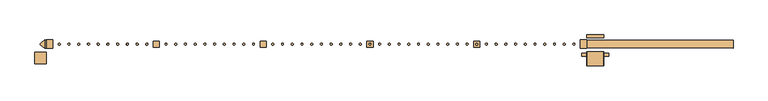
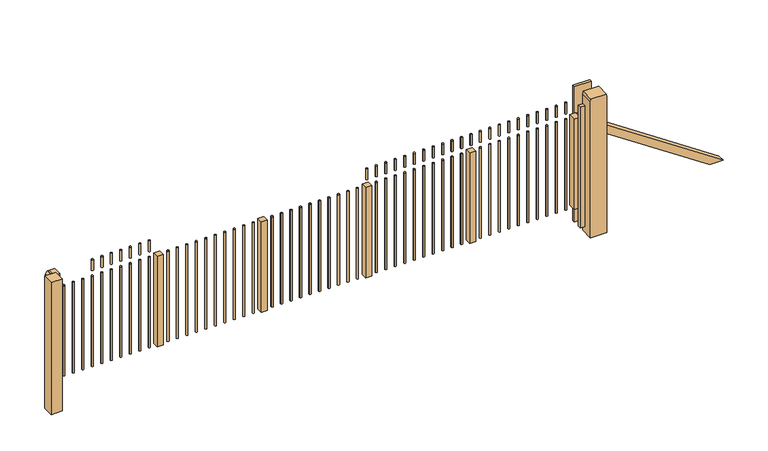
"""IFC4 building model written with IfcOpenShell, lengths in millimetres: door geometry, NLRS_90_DO_UN_schuifpoort met spijlen_gen_rsf : schuifpoort automatisch bxh 7000x1800-NP."""

import ifcopenshell
import ifcopenshell.guid

model = None  # the IFC model being written
_history = None  # IfcOwnerHistory: only IFC2X3 demands one
_inside = {}  # id of a spatial element -> (the spatial element, [elements in it])
_under = {}  # id of a project, library or spatial element -> (it, [spatial elements below it])
_declared = {}  # id of a project -> (the project, [libraries it declares])
_typed = {}  # id of a type object -> (the type object, [elements of that type])
_made_of = {}  # id of a material, layer set ... -> (it, [elements and type objects made of it])


def new_model(schema):
    """Start an empty IFC model of exactly this schema.

    Asked for "IFC4X3", IfcOpenShell would pick the latest addendum, in which some entities
    have other attributes; the version numbers below select the first issue.
    IFC2X3 requires an IfcOwnerHistory on every rooted entity: one is made here for all.
    """
    global model, _history
    if schema == "IFC4X3":
        model = ifcopenshell.file(schema_version=(4, 3, 0, 0))
    else:
        model = ifcopenshell.file(schema=schema)
    _inside.clear()
    _under.clear()
    _declared.clear()
    _typed.clear()
    _made_of.clear()
    _history = None
    if model.schema == "IFC2X3":
        org = make("IfcOrganization", Name="unknown")
        user = make(
            "IfcPersonAndOrganization",
            ThePerson=make("IfcPerson", FamilyName="unknown"),
            TheOrganization=org,
        )
        app = make(
            "IfcApplication",
            ApplicationDeveloper=org,
            Version="unknown",
            ApplicationFullName="unknown",
            ApplicationIdentifier="unknown",
        )
        _history = make(
            "IfcOwnerHistory",
            OwningUser=user,
            OwningApplication=app,
            ChangeAction="ADDED",
            CreationDate=0,
        )
    return model


def make(cls, **values):
    """One entity of the class cls with the attributes given. An attribute that is None is left unset."""
    return model.create_entity(
        cls, **{name: value for name, value in values.items() if value is not None}
    )


def rooted(cls, **values):
    """An entity with a GlobalId (a new one), such as an element, a storey or a relation."""
    return make(cls, GlobalId=ifcopenshell.guid.new(), OwnerHistory=_history, **values)


def si_unit(unit_type, name, prefix=None):
    """IfcSIUnit, for example si_unit("LENGTHUNIT", "METRE", prefix="MILLI")."""
    return make("IfcSIUnit", UnitType=unit_type, Prefix=prefix, Name=name)


def assignment(units):
    """IfcUnitAssignment: the units of a project."""
    return None if units is None else make("IfcUnitAssignment", Units=units)


def point(xyz):
    """IfcCartesianPoint."""
    return None if xyz is None else make("IfcCartesianPoint", Coordinates=xyz)


def direction(xyz):
    """IfcDirection."""
    return None if xyz is None else make("IfcDirection", DirectionRatios=xyz)


def frame(location, z_axis=None, x_axis=None):
    """IfcAxis2Placement3D, a coordinate frame: its origin and axes. An axis left out is left unset."""
    return make(
        "IfcAxis2Placement3D",
        Location=point(location),
        Axis=direction(z_axis),
        RefDirection=direction(x_axis),
    )


def frame_2d(location, x_axis=None):
    """IfcAxis2Placement2D, a coordinate frame in the plane: its origin and x axis."""
    return make(
        "IfcAxis2Placement2D", Location=point(location), RefDirection=direction(x_axis)
    )


def origin():
    """The frame at (0, 0, 0) with its axes left unset."""
    return frame((0.0, 0.0, 0.0))


def place(relative_to, where):
    """IfcLocalPlacement: puts the frame where relative to a parent placement (None: the world)."""
    return make(
        "IfcLocalPlacement", PlacementRelTo=relative_to, RelativePlacement=where
    )


def context(
    kind, dimensions, precision=None, world=None, true_north=None, identifier=None
):
    """IfcGeometricRepresentationContext, for example the 3D "Model" context."""
    return make(
        "IfcGeometricRepresentationContext",
        ContextIdentifier=identifier,
        ContextType=kind,
        CoordinateSpaceDimension=dimensions,
        Precision=precision,
        WorldCoordinateSystem=world,
        TrueNorth=true_north,
    )


def project(units=None, contexts=None):
    """IfcProject with its units and contexts."""
    return rooted(
        "IfcProject",
        Name="project",
        RepresentationContexts=contexts,
        UnitsInContext=assignment(units),
    )


def spatial(cls, under=None, at=None, **own):
    """A site, building, storey or space (cls), placed at a placement, below another one or the project."""
    s = rooted(cls, ObjectPlacement=at, **own)
    if under is not None:
        _under.setdefault(under.id(), (under, []))[1].append(s)
    return s


def polyline(points):
    """IfcPolyline through the points."""
    return make("IfcPolyline", Points=[point(p) for p in points])


def circle_curve(where, radius):
    """IfcCircle in the frame where."""
    return make("IfcCircle", Position=where, Radius=radius)


def trimmed(basis, trim1, trim2, sense, master):
    """IfcTrimmedCurve: the piece of a basis curve between two trims."""
    return make(
        "IfcTrimmedCurve",
        BasisCurve=basis,
        Trim1=trim1,
        Trim2=trim2,
        SenseAgreement=sense,
        MasterRepresentation=master,
    )


def segment(curve, same_sense, transition):
    """IfcCompositeCurveSegment."""
    return make(
        "IfcCompositeCurveSegment",
        Transition=transition,
        SameSense=same_sense,
        ParentCurve=curve,
    )


def composite_curve(segments, self_intersect=None):
    """IfcCompositeCurve: segments joined end to end."""
    return make("IfcCompositeCurve", Segments=segments, SelfIntersect=self_intersect)


def outline(outer, holes=None, kind="AREA"):
    """IfcArbitraryClosedProfileDef: a profile drawn as a closed curve; with holes, ...WithVoids."""
    if holes is None:
        return make("IfcArbitraryClosedProfileDef", ProfileType=kind, OuterCurve=outer)
    return make(
        "IfcArbitraryProfileDefWithVoids",
        ProfileType=kind,
        OuterCurve=outer,
        InnerCurves=holes,
    )


def extrude(swept, where, along, depth):
    """IfcExtrudedAreaSolid: the profile swept, set in the frame where, extruded along a direction by depth."""
    return make(
        "IfcExtrudedAreaSolid",
        SweptArea=swept,
        Position=where,
        ExtrudedDirection=direction(along),
        Depth=depth,
    )


def shape(context_of_items, identifier, shape_type, items):
    """IfcShapeRepresentation: the items that make up one representation, for example the "Body"."""
    return make(
        "IfcShapeRepresentation",
        ContextOfItems=context_of_items,
        RepresentationIdentifier=identifier,
        RepresentationType=shape_type,
        Items=items,
    )


def source(mapping_origin, context_of_items, identifier, shape_type, items):
    """IfcRepresentationMap: a shape defined once, which mapped items show again and again."""
    return make(
        "IfcRepresentationMap",
        MappingOrigin=mapping_origin,
        MappedRepresentation=shape(context_of_items, identifier, shape_type, items),
    )


def transform(
    local_origin,
    x_axis=None,
    y_axis=None,
    z_axis=None,
    scale=None,
    scale2=None,
    scale3=None,
    uniform=True,
):
    """IfcCartesianTransformationOperator3D, or its non-uniform kind. x_axis, y_axis, z_axis: its Axis1, 2, 3."""
    if uniform:
        return make(
            "IfcCartesianTransformationOperator3D",
            Axis1=direction(x_axis),
            Axis2=direction(y_axis),
            LocalOrigin=point(local_origin),
            Scale=scale,
            Axis3=direction(z_axis),
        )
    return make(
        "IfcCartesianTransformationOperator3DnonUniform",
        Axis1=direction(x_axis),
        Axis2=direction(y_axis),
        LocalOrigin=point(local_origin),
        Scale=scale,
        Axis3=direction(z_axis),
        Scale2=scale2,
        Scale3=scale3,
    )


def mapped(mapping_source, mapping_target):
    """IfcMappedItem: shows the shape of a source again, moved by a transform."""
    return make(
        "IfcMappedItem", MappingSource=mapping_source, MappingTarget=mapping_target
    )


def made_of(thing, what):
    """Note that an element or type object is made of a material, layer set ...; save() writes the relation."""
    if what is not None:
        _made_of.setdefault(what.id(), (what, []))[1].append(thing)
    return thing


def element(
    cls,
    number,
    at=None,
    inside=None,
    cuts=None,
    type_object=None,
    material=None,
    context=None,
    identifier="Body",
    shape_type=None,
    held_by="IfcProductDefinitionShape",
    body=None,
    shapes=None,
    **own,
):
    """One element of the class cls, such as IfcWall. Its Tag is "e" and its number.

    at: its placement. inside: the storey or other place that contains it. cuts: it is an
    opening in that element (IfcRelVoidsElement). A single representation is given by context,
    identifier, shape_type and body (its items); several are given by shapes. held_by: the class
    of the entity that holds the representations. save() writes the other relations.
    """
    e = rooted(cls, Tag="e%d" % number, ObjectPlacement=at, **own)
    if body is not None:
        shapes = [shape(context, identifier, shape_type, body)]
    if shapes is not None:
        e.Representation = make(held_by, Representations=shapes)
    if inside is not None:
        _inside.setdefault(inside.id(), (inside, []))[1].append(e)
    if cuts is not None:
        rooted(
            "IfcRelVoidsElement", RelatingBuildingElement=cuts, RelatedOpeningElement=e
        )
    if type_object is not None:
        _typed.setdefault(type_object.id(), (type_object, []))[1].append(e)
    return made_of(e, material)


def aggregate(whole, parts):
    """IfcRelAggregates: a whole, such as a stair, and the parts it consists of."""
    return rooted("IfcRelAggregates", RelatingObject=whole, RelatedObjects=parts)


def save(model, path):
    """Write the relations noted so far, then the file.

    IfcRelAggregates (storeys below a building ...), IfcRelContainedInSpatialStructure (elements
    in a storey), IfcRelDefinesByType, IfcRelAssociatesMaterial and IfcRelDeclares: one each for
    every whole, place, type object, material and project.
    """
    for whole, parts in _under.values():
        aggregate(whole, parts)
    for where, things in _inside.values():
        rooted(
            "IfcRelContainedInSpatialStructure",
            RelatedElements=things,
            RelatingStructure=where,
        )
    for kind, things in _typed.values():
        rooted("IfcRelDefinesByType", RelatedObjects=things, RelatingType=kind)
    for what, things in _made_of.values():
        rooted("IfcRelAssociatesMaterial", RelatedObjects=things, RelatingMaterial=what)
    for by, libraries in _declared.values():
        rooted("IfcRelDeclares", RelatingContext=by, RelatedDefinitions=libraries)
    model.write(path)


def door_c2b4a2f6(model_context):
    return source(origin(), model_context, "Body", "SweptSolid", [
        extrude(outline(composite_curve([segment(trimmed(circle_curve(frame_2d((3299.5, 0.0)), 12.5), [point((3312.0, 0.0))], [point((3287.0, 0.0))], False, "CARTESIAN"), True, "CONTINUOUS"), segment(trimmed(circle_curve(frame_2d((3299.5, 0.0)), 12.5), [point((3287.0, 0.0))], [point((3312.0, 0.0))], False, "CARTESIAN"), True, "CONTINUOUS")], self_intersect=False)), frame((0.0, 0.0, 300.0), z_axis=(0.0, 0.0, 1.0), x_axis=(1.0, 0.0, 0.0)), (0.0, 0.0, 1.0), 1270.0),
        extrude(outline(composite_curve([segment(trimmed(circle_curve(frame_2d((3173.5, 0.0)), 12.5), [point((3186.0, 0.0))], [point((3161.0, 0.0))], False, "CARTESIAN"), True, "CONTINUOUS"), segment(trimmed(circle_curve(frame_2d((3173.5, 0.0)), 12.5), [point((3161.0, 0.0))], [point((3186.0, 0.0))], False, "CARTESIAN"), True, "CONTINUOUS")], self_intersect=False)), frame((0.0, 0.0, 300.0), z_axis=(0.0, 0.0, 1.0), x_axis=(1.0, 0.0, 0.0)), (0.0, 0.0, 1.0), 1270.0),
        extrude(outline(composite_curve([segment(trimmed(circle_curve(frame_2d((3047.5, 0.0)), 12.5), [point((3060.0, 0.0))], [point((3035.0, 0.0))], False, "CARTESIAN"), True, "CONTINUOUS"), segment(trimmed(circle_curve(frame_2d((3047.5, 0.0)), 12.5), [point((3035.0, 0.0))], [point((3060.0, 0.0))], False, "CARTESIAN"), True, "CONTINUOUS")], self_intersect=False)), frame((0.0, 0.0, 300.0), z_axis=(0.0, 0.0, 1.0), x_axis=(1.0, 0.0, 0.0)), (0.0, 0.0, 1.0), 1270.0),
        extrude(outline(composite_curve([segment(trimmed(circle_curve(frame_2d((2921.5, 0.0)), 12.5), [point((2934.0, 0.0))], [point((2909.0, 0.0))], False, "CARTESIAN"), True, "CONTINUOUS"), segment(trimmed(circle_curve(frame_2d((2921.5, 0.0)), 12.5), [point((2909.0, 0.0))], [point((2934.0, 0.0))], False, "CARTESIAN"), True, "CONTINUOUS")], self_intersect=False)), frame((0.0, 0.0, 300.0), z_axis=(0.0, 0.0, 1.0), x_axis=(1.0, 0.0, 0.0)), (0.0, 0.0, 1.0), 1270.0),
        extrude(outline(composite_curve([segment(trimmed(circle_curve(frame_2d((2795.5, 0.0)), 12.5), [point((2808.0, 0.0))], [point((2783.0, 0.0))], False, "CARTESIAN"), True, "CONTINUOUS"), segment(trimmed(circle_curve(frame_2d((2795.5, 0.0)), 12.5), [point((2783.0, 0.0))], [point((2808.0, 0.0))], False, "CARTESIAN"), True, "CONTINUOUS")], self_intersect=False)), frame((0.0, 0.0, 300.0), z_axis=(0.0, 0.0, 1.0), x_axis=(1.0, 0.0, 0.0)), (0.0, 0.0, 1.0), 1270.0),
        extrude(outline(composite_curve([segment(trimmed(circle_curve(frame_2d((2669.5, 0.0)), 12.5), [point((2682.0, 0.0))], [point((2657.0, 0.0))], False, "CARTESIAN"), True, "CONTINUOUS"), segment(trimmed(circle_curve(frame_2d((2669.5, 0.0)), 12.5), [point((2657.0, 0.0))], [point((2682.0, 0.0))], False, "CARTESIAN"), True, "CONTINUOUS")], self_intersect=False)), frame((0.0, 0.0, 300.0), z_axis=(0.0, 0.0, 1.0), x_axis=(1.0, 0.0, 0.0)), (0.0, 0.0, 1.0), 1270.0),
        extrude(outline(composite_curve([segment(trimmed(circle_curve(frame_2d((2543.5, 0.0)), 12.5), [point((2556.0, 0.0))], [point((2531.0, 0.0))], False, "CARTESIAN"), True, "CONTINUOUS"), segment(trimmed(circle_curve(frame_2d((2543.5, 0.0)), 12.5), [point((2531.0, 0.0))], [point((2556.0, 0.0))], False, "CARTESIAN"), True, "CONTINUOUS")], self_intersect=False)), frame((0.0, 0.0, 300.0), z_axis=(0.0, 0.0, 1.0), x_axis=(1.0, 0.0, 0.0)), (0.0, 0.0, 1.0), 1270.0),
        extrude(outline(composite_curve([segment(trimmed(circle_curve(frame_2d((2417.5, 0.0)), 12.5), [point((2430.0, 0.0))], [point((2405.0, 0.0))], False, "CARTESIAN"), True, "CONTINUOUS"), segment(trimmed(circle_curve(frame_2d((2417.5, 0.0)), 12.5), [point((2405.0, 0.0))], [point((2430.0, 0.0))], False, "CARTESIAN"), True, "CONTINUOUS")], self_intersect=False)), frame((0.0, 0.0, 300.0), z_axis=(0.0, 0.0, 1.0), x_axis=(1.0, 0.0, 0.0)), (0.0, 0.0, 1.0), 1270.0),
        extrude(outline(composite_curve([segment(trimmed(circle_curve(frame_2d((2291.5, 0.0)), 12.5), [point((2304.0, 0.0))], [point((2279.0, 0.0))], False, "CARTESIAN"), True, "CONTINUOUS"), segment(trimmed(circle_curve(frame_2d((2291.5, 0.0)), 12.5), [point((2279.0, 0.0))], [point((2304.0, 0.0))], False, "CARTESIAN"), True, "CONTINUOUS")], self_intersect=False)), frame((0.0, 0.0, 300.0), z_axis=(0.0, 0.0, 1.0), x_axis=(1.0, 0.0, 0.0)), (0.0, 0.0, 1.0), 1270.0),
        extrude(outline(composite_curve([segment(trimmed(circle_curve(frame_2d((2165.5, 0.0)), 12.5), [point((2178.0, 0.0))], [point((2153.0, 0.0))], False, "CARTESIAN"), True, "CONTINUOUS"), segment(trimmed(circle_curve(frame_2d((2165.5, 0.0)), 12.5), [point((2153.0, 0.0))], [point((2178.0, 0.0))], False, "CARTESIAN"), True, "CONTINUOUS")], self_intersect=False)), frame((0.0, 0.0, 300.0), z_axis=(0.0, 0.0, 1.0), x_axis=(1.0, 0.0, 0.0)), (0.0, 0.0, 1.0), 1270.0),
        extrude(outline(composite_curve([segment(trimmed(circle_curve(frame_2d((1915.5, 0.0)), 12.5), [point((1928.0, 0.0))], [point((1903.0, 0.0))], False, "CARTESIAN"), True, "CONTINUOUS"), segment(trimmed(circle_curve(frame_2d((1915.5, 0.0)), 12.5), [point((1903.0, 0.0))], [point((1928.0, 0.0))], False, "CARTESIAN"), True, "CONTINUOUS")], self_intersect=False)), frame((0.0, 0.0, 300.0), z_axis=(0.0, 0.0, 1.0), x_axis=(1.0, 0.0, 0.0)), (0.0, 0.0, 1.0), 1270.0),
        extrude(outline(composite_curve([segment(trimmed(circle_curve(frame_2d((1789.5, 0.0)), 12.5), [point((1802.0, 0.0))], [point((1777.0, 0.0))], False, "CARTESIAN"), True, "CONTINUOUS"), segment(trimmed(circle_curve(frame_2d((1789.5, 0.0)), 12.5), [point((1777.0, 0.0))], [point((1802.0, 0.0))], False, "CARTESIAN"), True, "CONTINUOUS")], self_intersect=False)), frame((0.0, 0.0, 300.0), z_axis=(0.0, 0.0, 1.0), x_axis=(1.0, 0.0, 0.0)), (0.0, 0.0, 1.0), 1270.0),
        extrude(outline(composite_curve([segment(trimmed(circle_curve(frame_2d((1663.5, 0.0)), 12.5), [point((1676.0, 0.0))], [point((1651.0, 0.0))], False, "CARTESIAN"), True, "CONTINUOUS"), segment(trimmed(circle_curve(frame_2d((1663.5, 0.0)), 12.5), [point((1651.0, 0.0))], [point((1676.0, 0.0))], False, "CARTESIAN"), True, "CONTINUOUS")], self_intersect=False)), frame((0.0, 0.0, 300.0), z_axis=(0.0, 0.0, 1.0), x_axis=(1.0, 0.0, 0.0)), (0.0, 0.0, 1.0), 1270.0),
        extrude(outline(composite_curve([segment(trimmed(circle_curve(frame_2d((1537.5, 0.0)), 12.5), [point((1550.0, 0.0))], [point((1525.0, 0.0))], False, "CARTESIAN"), True, "CONTINUOUS"), segment(trimmed(circle_curve(frame_2d((1537.5, 0.0)), 12.5), [point((1525.0, 0.0))], [point((1550.0, 0.0))], False, "CARTESIAN"), True, "CONTINUOUS")], self_intersect=False)), frame((0.0, 0.0, 300.0), z_axis=(0.0, 0.0, 1.0), x_axis=(1.0, 0.0, 0.0)), (0.0, 0.0, 1.0), 1270.0),
        extrude(outline(composite_curve([segment(trimmed(circle_curve(frame_2d((1411.5, 0.0)), 12.5), [point((1424.0, 0.0))], [point((1399.0, 0.0))], False, "CARTESIAN"), True, "CONTINUOUS"), segment(trimmed(circle_curve(frame_2d((1411.5, 0.0)), 12.5), [point((1399.0, 0.0))], [point((1424.0, 0.0))], False, "CARTESIAN"), True, "CONTINUOUS")], self_intersect=False)), frame((0.0, 0.0, 300.0), z_axis=(0.0, 0.0, 1.0), x_axis=(1.0, 0.0, 0.0)), (0.0, 0.0, 1.0), 1270.0),
        extrude(outline(composite_curve([segment(trimmed(circle_curve(frame_2d((1285.5, 0.0)), 12.5), [point((1298.0, 0.0))], [point((1273.0, 0.0))], False, "CARTESIAN"), True, "CONTINUOUS"), segment(trimmed(circle_curve(frame_2d((1285.5, 0.0)), 12.5), [point((1273.0, 0.0))], [point((1298.0, 0.0))], False, "CARTESIAN"), True, "CONTINUOUS")], self_intersect=False)), frame((0.0, 0.0, 300.0), z_axis=(0.0, 0.0, 1.0), x_axis=(1.0, 0.0, 0.0)), (0.0, 0.0, 1.0), 1270.0),
        extrude(outline(composite_curve([segment(trimmed(circle_curve(frame_2d((1159.5, 0.0)), 12.5), [point((1172.0, 0.0))], [point((1147.0, 0.0))], False, "CARTESIAN"), True, "CONTINUOUS"), segment(trimmed(circle_curve(frame_2d((1159.5, 0.0)), 12.5), [point((1147.0, 0.0))], [point((1172.0, 0.0))], False, "CARTESIAN"), True, "CONTINUOUS")], self_intersect=False)), frame((0.0, 0.0, 300.0), z_axis=(0.0, 0.0, 1.0), x_axis=(1.0, 0.0, 0.0)), (0.0, 0.0, 1.0), 1270.0),
        extrude(outline(composite_curve([segment(trimmed(circle_curve(frame_2d((1033.5, 0.0)), 12.5), [point((1046.0, 0.0))], [point((1021.0, 0.0))], False, "CARTESIAN"), True, "CONTINUOUS"), segment(trimmed(circle_curve(frame_2d((1033.5, 0.0)), 12.5), [point((1021.0, 0.0))], [point((1046.0, 0.0))], False, "CARTESIAN"), True, "CONTINUOUS")], self_intersect=False)), frame((0.0, 0.0, 300.0), z_axis=(0.0, 0.0, 1.0), x_axis=(1.0, 0.0, 0.0)), (0.0, 0.0, 1.0), 1270.0),
        extrude(outline(composite_curve([segment(trimmed(circle_curve(frame_2d((907.5, 0.0)), 12.5), [point((920.0, 0.0))], [point((895.0, 0.0))], False, "CARTESIAN"), True, "CONTINUOUS"), segment(trimmed(circle_curve(frame_2d((907.5, 0.0)), 12.5), [point((895.0, 0.0))], [point((920.0, 0.0))], False, "CARTESIAN"), True, "CONTINUOUS")], self_intersect=False)), frame((0.0, 0.0, 300.0), z_axis=(0.0, 0.0, 1.0), x_axis=(1.0, 0.0, 0.0)), (0.0, 0.0, 1.0), 1270.0),
        extrude(outline(composite_curve([segment(trimmed(circle_curve(frame_2d((781.5, 0.0)), 12.5), [point((794.0, 0.0))], [point((769.0, 0.0))], False, "CARTESIAN"), True, "CONTINUOUS"), segment(trimmed(circle_curve(frame_2d((781.5, 0.0)), 12.5), [point((769.0, 0.0))], [point((794.0, 0.0))], False, "CARTESIAN"), True, "CONTINUOUS")], self_intersect=False)), frame((0.0, 0.0, 300.0), z_axis=(0.0, 0.0, 1.0), x_axis=(1.0, 0.0, 0.0)), (0.0, 0.0, 1.0), 1270.0),
        extrude(outline(polyline([(3465.0, -158.5), (3400.0, -158.5), (3400.0, -118.5), (3465.0, -118.5), (3465.0, -158.5)])), frame((0.0, 0.0, 100.0), z_axis=(0.0, 0.0, 1.0), x_axis=(1.0, 0.0, 0.0)), (0.0, 0.0, 1.0), 1700.0),
        extrude(outline(polyline([(3685.0, -158.5), (3685.0, -118.5), (3750.0, -118.5), (3750.0, -158.5), (3685.0, -158.5)])), frame((0.0, 0.0, 100.0), z_axis=(0.0, 0.0, 1.0), x_axis=(1.0, 0.0, 0.0)), (0.0, 0.0, 1.0), 1700.0),
        extrude(outline(polyline([(3685.0, 84.5), (3465.0, 84.5), (3465.0, 119.5), (3685.0, 119.5), (3685.0, 84.5)])), frame((0.0, 0.0, 12.0), z_axis=(0.0, 0.0, 1.0), x_axis=(1.0, 0.0, 0.0)), (0.0, 0.0, 1.0), 1906.0),
        extrude(outline(polyline([(1918.0, 3465.0), (12.0, 3465.0), (12.0, 3685.0), (1918.0, 3685.0), (1960.0, 3677.5), (1960.0, 3472.5), (1918.0, 3465.0)])), frame((0.0, -280.5, 0.0), z_axis=(0.0, 1.0, 0.0), x_axis=(0.0, 0.0, 1.0)), (0.0, 0.0, 1.0), 180.0),
        extrude(outline(polyline([(2000.5, -40.0), (2000.5, 40.0), (2080.5, 40.0), (2080.5, -40.0), (2000.5, -40.0)])), frame((0.0, 0.0, 300.0), z_axis=(0.0, 0.0, 1.0), x_axis=(1.0, 0.0, 0.0)), (0.0, 0.0, 1.0), 1270.0),
        extrude(outline(polyline([(616.5, -40.0), (616.5, 40.0), (696.5, 40.0), (696.5, -40.0), (616.5, -40.0)])), frame((0.0, 0.0, 300.0), z_axis=(0.0, 0.0, 1.0), x_axis=(1.0, 0.0, 0.0)), (0.0, 0.0, 1.0), 1270.0),
        extrude(outline(polyline([(-767.5, -40.0), (-767.5, 40.0), (-687.5, 40.0), (-687.5, -40.0), (-767.5, -40.0)])), frame((0.0, 0.0, 300.0), z_axis=(0.0, 0.0, 1.0), x_axis=(1.0, 0.0, 0.0)), (0.0, 0.0, 1.0), 1270.0),
        extrude(outline(polyline([(-2151.5, -40.0), (-2151.5, 40.0), (-2071.5, 40.0), (-2071.5, -40.0), (-2151.5, -40.0)])), frame((0.0, 0.0, 300.0), z_axis=(0.0, 0.0, 1.0), x_axis=(1.0, 0.0, 0.0)), (0.0, 0.0, 1.0), 1270.0),
        extrude(outline(composite_curve([segment(trimmed(circle_curve(frame_2d((531.5, 0.0)), 12.5), [point((544.0, 0.0))], [point((519.0, 0.0))], False, "CARTESIAN"), True, "CONTINUOUS"), segment(trimmed(circle_curve(frame_2d((531.5, 0.0)), 12.5), [point((519.0, 0.0))], [point((544.0, 0.0))], False, "CARTESIAN"), True, "CONTINUOUS")], self_intersect=False)), frame((0.0, 0.0, 300.0), z_axis=(0.0, 0.0, 1.0), x_axis=(1.0, 0.0, 0.0)), (0.0, 0.0, 1.0), 1270.0),
        extrude(outline(composite_curve([segment(trimmed(circle_curve(frame_2d((405.5, 0.0)), 12.5), [point((418.0, 0.0))], [point((393.0, 0.0))], False, "CARTESIAN"), True, "CONTINUOUS"), segment(trimmed(circle_curve(frame_2d((405.5, 0.0)), 12.5), [point((393.0, 0.0))], [point((418.0, 0.0))], False, "CARTESIAN"), True, "CONTINUOUS")], self_intersect=False)), frame((0.0, 0.0, 300.0), z_axis=(0.0, 0.0, 1.0), x_axis=(1.0, 0.0, 0.0)), (0.0, 0.0, 1.0), 1270.0),
        extrude(outline(composite_curve([segment(trimmed(circle_curve(frame_2d((279.5, 0.0)), 12.5), [point((292.0, 0.0))], [point((267.0, 0.0))], False, "CARTESIAN"), True, "CONTINUOUS"), segment(trimmed(circle_curve(frame_2d((279.5, 0.0)), 12.5), [point((267.0, 0.0))], [point((292.0, 0.0))], False, "CARTESIAN"), True, "CONTINUOUS")], self_intersect=False)), frame((0.0, 0.0, 300.0), z_axis=(0.0, 0.0, 1.0), x_axis=(1.0, 0.0, 0.0)), (0.0, 0.0, 1.0), 1270.0),
        extrude(outline(composite_curve([segment(trimmed(circle_curve(frame_2d((153.5, 0.0)), 12.5), [point((166.0, 0.0))], [point((141.0, 0.0))], False, "CARTESIAN"), True, "CONTINUOUS"), segment(trimmed(circle_curve(frame_2d((153.5, 0.0)), 12.5), [point((141.0, 0.0))], [point((166.0, 0.0))], False, "CARTESIAN"), True, "CONTINUOUS")], self_intersect=False)), frame((0.0, 0.0, 300.0), z_axis=(0.0, 0.0, 1.0), x_axis=(1.0, 0.0, 0.0)), (0.0, 0.0, 1.0), 1270.0),
        extrude(outline(composite_curve([segment(trimmed(circle_curve(frame_2d((27.5, 0.0)), 12.5), [point((40.0, 0.0))], [point((15.0, 0.0))], False, "CARTESIAN"), True, "CONTINUOUS"), segment(trimmed(circle_curve(frame_2d((27.5, 0.0)), 12.5), [point((15.0, 0.0))], [point((40.0, 0.0))], False, "CARTESIAN"), True, "CONTINUOUS")], self_intersect=False)), frame((0.0, 0.0, 300.0), z_axis=(0.0, 0.0, 1.0), x_axis=(1.0, 0.0, 0.0)), (0.0, 0.0, 1.0), 1270.0),
        extrude(outline(composite_curve([segment(trimmed(circle_curve(frame_2d((-98.5, 0.0)), 12.5), [point((-86.0, 0.0))], [point((-111.0, 0.0))], False, "CARTESIAN"), True, "CONTINUOUS"), segment(trimmed(circle_curve(frame_2d((-98.5, 0.0)), 12.5), [point((-111.0, 0.0))], [point((-86.0, 0.0))], False, "CARTESIAN"), True, "CONTINUOUS")], self_intersect=False)), frame((0.0, 0.0, 300.0), z_axis=(0.0, 0.0, 1.0), x_axis=(1.0, 0.0, 0.0)), (0.0, 0.0, 1.0), 1270.0),
        extrude(outline(composite_curve([segment(trimmed(circle_curve(frame_2d((-224.5, 0.0)), 12.5), [point((-212.0, 0.0))], [point((-237.0, 0.0))], False, "CARTESIAN"), True, "CONTINUOUS"), segment(trimmed(circle_curve(frame_2d((-224.5, 0.0)), 12.5), [point((-237.0, 0.0))], [point((-212.0, 0.0))], False, "CARTESIAN"), True, "CONTINUOUS")], self_intersect=False)), frame((0.0, 0.0, 300.0), z_axis=(0.0, 0.0, 1.0), x_axis=(1.0, 0.0, 0.0)), (0.0, 0.0, 1.0), 1270.0),
        extrude(outline(composite_curve([segment(trimmed(circle_curve(frame_2d((-350.5, 0.0)), 12.5), [point((-338.0, 0.0))], [point((-363.0, 0.0))], False, "CARTESIAN"), True, "CONTINUOUS"), segment(trimmed(circle_curve(frame_2d((-350.5, 0.0)), 12.5), [point((-363.0, 0.0))], [point((-338.0, 0.0))], False, "CARTESIAN"), True, "CONTINUOUS")], self_intersect=False)), frame((0.0, 0.0, 300.0), z_axis=(0.0, 0.0, 1.0), x_axis=(1.0, 0.0, 0.0)), (0.0, 0.0, 1.0), 1270.0),
        extrude(outline(composite_curve([segment(trimmed(circle_curve(frame_2d((-476.5, 0.0)), 12.5), [point((-464.0, 0.0))], [point((-489.0, 0.0))], False, "CARTESIAN"), True, "CONTINUOUS"), segment(trimmed(circle_curve(frame_2d((-476.5, 0.0)), 12.5), [point((-489.0, 0.0))], [point((-464.0, 0.0))], False, "CARTESIAN"), True, "CONTINUOUS")], self_intersect=False)), frame((0.0, 0.0, 300.0), z_axis=(0.0, 0.0, 1.0), x_axis=(1.0, 0.0, 0.0)), (0.0, 0.0, 1.0), 1270.0),
        extrude(outline(composite_curve([segment(trimmed(circle_curve(frame_2d((-602.5, 0.0)), 12.5), [point((-590.0, 0.0))], [point((-615.0, 0.0))], False, "CARTESIAN"), True, "CONTINUOUS"), segment(trimmed(circle_curve(frame_2d((-602.5, 0.0)), 12.5), [point((-615.0, 0.0))], [point((-590.0, 0.0))], False, "CARTESIAN"), True, "CONTINUOUS")], self_intersect=False)), frame((0.0, 0.0, 300.0), z_axis=(0.0, 0.0, 1.0), x_axis=(1.0, 0.0, 0.0)), (0.0, 0.0, 1.0), 1270.0),
        extrude(outline(polyline([(300.0, 5362.0), (1570.0, 3464.5), (1449.6685917, 3464.5), (300.0, 5182.2135061), (300.0, 5362.0)])), frame((0.0, -50.0, 0.0), z_axis=(0.0, 1.0, 0.0), x_axis=(0.0, 0.0, 1.0)), (0.0, 0.0, 1.0), 100.0),
        extrude(outline(composite_curve([segment(trimmed(circle_curve(frame_2d((-852.5, 0.0)), 12.5), [point((-840.0, 0.0))], [point((-865.0, 0.0))], False, "CARTESIAN"), True, "CONTINUOUS"), segment(trimmed(circle_curve(frame_2d((-852.5, 0.0)), 12.5), [point((-865.0, 0.0))], [point((-840.0, 0.0))], False, "CARTESIAN"), True, "CONTINUOUS")], self_intersect=False)), frame((0.0, 0.0, 300.0), z_axis=(0.0, 0.0, 1.0), x_axis=(1.0, 0.0, 0.0)), (0.0, 0.0, 1.0), 1270.0),
        extrude(outline(composite_curve([segment(trimmed(circle_curve(frame_2d((-978.5, 0.0)), 12.5), [point((-966.0, 0.0))], [point((-991.0, 0.0))], False, "CARTESIAN"), True, "CONTINUOUS"), segment(trimmed(circle_curve(frame_2d((-978.5, 0.0)), 12.5), [point((-991.0, 0.0))], [point((-966.0, 0.0))], False, "CARTESIAN"), True, "CONTINUOUS")], self_intersect=False)), frame((0.0, 0.0, 300.0), z_axis=(0.0, 0.0, 1.0), x_axis=(1.0, 0.0, 0.0)), (0.0, 0.0, 1.0), 1270.0),
        extrude(outline(composite_curve([segment(trimmed(circle_curve(frame_2d((-1104.5, 0.0)), 12.5), [point((-1092.0, 0.0))], [point((-1117.0, 0.0))], False, "CARTESIAN"), True, "CONTINUOUS"), segment(trimmed(circle_curve(frame_2d((-1104.5, 0.0)), 12.5), [point((-1117.0, 0.0))], [point((-1092.0, 0.0))], False, "CARTESIAN"), True, "CONTINUOUS")], self_intersect=False)), frame((0.0, 0.0, 300.0), z_axis=(0.0, 0.0, 1.0), x_axis=(1.0, 0.0, 0.0)), (0.0, 0.0, 1.0), 1270.0),
        extrude(outline(composite_curve([segment(trimmed(circle_curve(frame_2d((-1230.5, 0.0)), 12.5), [point((-1218.0, 0.0))], [point((-1243.0, 0.0))], False, "CARTESIAN"), True, "CONTINUOUS"), segment(trimmed(circle_curve(frame_2d((-1230.5, 0.0)), 12.5), [point((-1243.0, 0.0))], [point((-1218.0, 0.0))], False, "CARTESIAN"), True, "CONTINUOUS")], self_intersect=False)), frame((0.0, 0.0, 300.0), z_axis=(0.0, 0.0, 1.0), x_axis=(1.0, 0.0, 0.0)), (0.0, 0.0, 1.0), 1270.0),
        extrude(outline(composite_curve([segment(trimmed(circle_curve(frame_2d((-1356.5, 0.0)), 12.5), [point((-1344.0, 0.0))], [point((-1369.0, 0.0))], False, "CARTESIAN"), True, "CONTINUOUS"), segment(trimmed(circle_curve(frame_2d((-1356.5, 0.0)), 12.5), [point((-1369.0, 0.0))], [point((-1344.0, 0.0))], False, "CARTESIAN"), True, "CONTINUOUS")], self_intersect=False)), frame((0.0, 0.0, 300.0), z_axis=(0.0, 0.0, 1.0), x_axis=(1.0, 0.0, 0.0)), (0.0, 0.0, 1.0), 1270.0),
        extrude(outline(composite_curve([segment(trimmed(circle_curve(frame_2d((-1482.5, 0.0)), 12.5), [point((-1470.0, 0.0))], [point((-1495.0, 0.0))], False, "CARTESIAN"), True, "CONTINUOUS"), segment(trimmed(circle_curve(frame_2d((-1482.5, 0.0)), 12.5), [point((-1495.0, 0.0))], [point((-1470.0, 0.0))], False, "CARTESIAN"), True, "CONTINUOUS")], self_intersect=False)), frame((0.0, 0.0, 300.0), z_axis=(0.0, 0.0, 1.0), x_axis=(1.0, 0.0, 0.0)), (0.0, 0.0, 1.0), 1270.0),
        extrude(outline(composite_curve([segment(trimmed(circle_curve(frame_2d((-1608.5, 0.0)), 12.5), [point((-1596.0, 0.0))], [point((-1621.0, 0.0))], False, "CARTESIAN"), True, "CONTINUOUS"), segment(trimmed(circle_curve(frame_2d((-1608.5, 0.0)), 12.5), [point((-1621.0, 0.0))], [point((-1596.0, 0.0))], False, "CARTESIAN"), True, "CONTINUOUS")], self_intersect=False)), frame((0.0, 0.0, 300.0), z_axis=(0.0, 0.0, 1.0), x_axis=(1.0, 0.0, 0.0)), (0.0, 0.0, 1.0), 1270.0),
        extrude(outline(composite_curve([segment(trimmed(circle_curve(frame_2d((-1734.5, 0.0)), 12.5), [point((-1722.0, 0.0))], [point((-1747.0, 0.0))], False, "CARTESIAN"), True, "CONTINUOUS"), segment(trimmed(circle_curve(frame_2d((-1734.5, 0.0)), 12.5), [point((-1747.0, 0.0))], [point((-1722.0, 0.0))], False, "CARTESIAN"), True, "CONTINUOUS")], self_intersect=False)), frame((0.0, 0.0, 300.0), z_axis=(0.0, 0.0, 1.0), x_axis=(1.0, 0.0, 0.0)), (0.0, 0.0, 1.0), 1270.0),
        extrude(outline(composite_curve([segment(trimmed(circle_curve(frame_2d((-1860.5, 0.0)), 12.5), [point((-1848.0, 0.0))], [point((-1873.0, 0.0))], False, "CARTESIAN"), True, "CONTINUOUS"), segment(trimmed(circle_curve(frame_2d((-1860.5, 0.0)), 12.5), [point((-1873.0, 0.0))], [point((-1848.0, 0.0))], False, "CARTESIAN"), True, "CONTINUOUS")], self_intersect=False)), frame((0.0, 0.0, 300.0), z_axis=(0.0, 0.0, 1.0), x_axis=(1.0, 0.0, 0.0)), (0.0, 0.0, 1.0), 1270.0),
        extrude(outline(composite_curve([segment(trimmed(circle_curve(frame_2d((-1986.5, 0.0)), 12.5), [point((-1974.0, 0.0))], [point((-1999.0, 0.0))], False, "CARTESIAN"), True, "CONTINUOUS"), segment(trimmed(circle_curve(frame_2d((-1986.5, 0.0)), 12.5), [point((-1999.0, 0.0))], [point((-1974.0, 0.0))], False, "CARTESIAN"), True, "CONTINUOUS")], self_intersect=False)), frame((0.0, 0.0, 300.0), z_axis=(0.0, 0.0, 1.0), x_axis=(1.0, 0.0, 0.0)), (0.0, 0.0, 1.0), 1270.0),
        extrude(outline(composite_curve([segment(trimmed(circle_curve(frame_2d((-2236.0, 0.0)), 12.5), [point((-2223.5, 0.0))], [point((-2248.5, 0.0))], False, "CARTESIAN"), True, "CONTINUOUS"), segment(trimmed(circle_curve(frame_2d((-2236.0, 0.0)), 12.5), [point((-2248.5, 0.0))], [point((-2223.5, 0.0))], False, "CARTESIAN"), True, "CONTINUOUS")], self_intersect=False)), frame((0.0, 0.0, 300.0), z_axis=(0.0, 0.0, 1.0), x_axis=(1.0, 0.0, 0.0)), (0.0, 0.0, 1.0), 1270.0),
        extrude(outline(composite_curve([segment(trimmed(circle_curve(frame_2d((-2362.0, 0.0)), 12.5), [point((-2349.5, 0.0))], [point((-2374.5, 0.0))], False, "CARTESIAN"), True, "CONTINUOUS"), segment(trimmed(circle_curve(frame_2d((-2362.0, 0.0)), 12.5), [point((-2374.5, 0.0))], [point((-2349.5, 0.0))], False, "CARTESIAN"), True, "CONTINUOUS")], self_intersect=False)), frame((0.0, 0.0, 300.0), z_axis=(0.0, 0.0, 1.0), x_axis=(1.0, 0.0, 0.0)), (0.0, 0.0, 1.0), 1270.0),
        extrude(outline(composite_curve([segment(trimmed(circle_curve(frame_2d((-2488.0, 0.0)), 12.5), [point((-2475.5, 0.0))], [point((-2500.5, 0.0))], False, "CARTESIAN"), True, "CONTINUOUS"), segment(trimmed(circle_curve(frame_2d((-2488.0, 0.0)), 12.5), [point((-2500.5, 0.0))], [point((-2475.5, 0.0))], False, "CARTESIAN"), True, "CONTINUOUS")], self_intersect=False)), frame((0.0, 0.0, 300.0), z_axis=(0.0, 0.0, 1.0), x_axis=(1.0, 0.0, 0.0)), (0.0, 0.0, 1.0), 1270.0),
        extrude(outline(composite_curve([segment(trimmed(circle_curve(frame_2d((-2614.0, 0.0)), 12.5), [point((-2601.5, 0.0))], [point((-2626.5, 0.0))], False, "CARTESIAN"), True, "CONTINUOUS"), segment(trimmed(circle_curve(frame_2d((-2614.0, 0.0)), 12.5), [point((-2626.5, 0.0))], [point((-2601.5, 0.0))], False, "CARTESIAN"), True, "CONTINUOUS")], self_intersect=False)), frame((0.0, 0.0, 300.0), z_axis=(0.0, 0.0, 1.0), x_axis=(1.0, 0.0, 0.0)), (0.0, 0.0, 1.0), 1270.0),
        extrude(outline(composite_curve([segment(trimmed(circle_curve(frame_2d((-2740.0, 0.0)), 12.5), [point((-2727.5, 0.0))], [point((-2752.5, 0.0))], False, "CARTESIAN"), True, "CONTINUOUS"), segment(trimmed(circle_curve(frame_2d((-2740.0, 0.0)), 12.5), [point((-2752.5, 0.0))], [point((-2727.5, 0.0))], False, "CARTESIAN"), True, "CONTINUOUS")], self_intersect=False)), frame((0.0, 0.0, 300.0), z_axis=(0.0, 0.0, 1.0), x_axis=(1.0, 0.0, 0.0)), (0.0, 0.0, 1.0), 1270.0),
        extrude(outline(composite_curve([segment(trimmed(circle_curve(frame_2d((-2866.0, 0.0)), 12.5), [point((-2853.5, 0.0))], [point((-2878.5, 0.0))], False, "CARTESIAN"), True, "CONTINUOUS"), segment(trimmed(circle_curve(frame_2d((-2866.0, 0.0)), 12.5), [point((-2878.5, 0.0))], [point((-2853.5, 0.0))], False, "CARTESIAN"), True, "CONTINUOUS")], self_intersect=False)), frame((0.0, 0.0, 300.0), z_axis=(0.0, 0.0, 1.0), x_axis=(1.0, 0.0, 0.0)), (0.0, 0.0, 1.0), 1270.0),
        extrude(outline(composite_curve([segment(trimmed(circle_curve(frame_2d((-2992.0, 0.0)), 12.5), [point((-2979.5, 0.0))], [point((-3004.5, 0.0))], False, "CARTESIAN"), True, "CONTINUOUS"), segment(trimmed(circle_curve(frame_2d((-2992.0, 0.0)), 12.5), [point((-3004.5, 0.0))], [point((-2979.5, 0.0))], False, "CARTESIAN"), True, "CONTINUOUS")], self_intersect=False)), frame((0.0, 0.0, 300.0), z_axis=(0.0, 0.0, 1.0), x_axis=(1.0, 0.0, 0.0)), (0.0, 0.0, 1.0), 1270.0),
        extrude(outline(composite_curve([segment(trimmed(circle_curve(frame_2d((-3118.0, 0.0)), 12.5), [point((-3105.5, 0.0))], [point((-3130.5, 0.0))], False, "CARTESIAN"), True, "CONTINUOUS"), segment(trimmed(circle_curve(frame_2d((-3118.0, 0.0)), 12.5), [point((-3130.5, 0.0))], [point((-3105.5, 0.0))], False, "CARTESIAN"), True, "CONTINUOUS")], self_intersect=False)), frame((0.0, 0.0, 300.0), z_axis=(0.0, 0.0, 1.0), x_axis=(1.0, 0.0, 0.0)), (0.0, 0.0, 1.0), 1270.0),
        extrude(outline(composite_curve([segment(trimmed(circle_curve(frame_2d((-3244.0, 0.0)), 12.5), [point((-3231.5, 0.0))], [point((-3256.5, 0.0))], False, "CARTESIAN"), True, "CONTINUOUS"), segment(trimmed(circle_curve(frame_2d((-3244.0, 0.0)), 12.5), [point((-3256.5, 0.0))], [point((-3231.5, 0.0))], False, "CARTESIAN"), True, "CONTINUOUS")], self_intersect=False)), frame((0.0, 0.0, 300.0), z_axis=(0.0, 0.0, 1.0), x_axis=(1.0, 0.0, 0.0)), (0.0, 0.0, 1.0), 1270.0),
        extrude(outline(composite_curve([segment(trimmed(circle_curve(frame_2d((-3370.0, 0.0)), 12.5), [point((-3357.5, 0.0))], [point((-3382.5, 0.0))], False, "CARTESIAN"), True, "CONTINUOUS"), segment(trimmed(circle_curve(frame_2d((-3370.0, 0.0)), 12.5), [point((-3382.5, 0.0))], [point((-3357.5, 0.0))], False, "CARTESIAN"), True, "CONTINUOUS")], self_intersect=False)), frame((0.0, 0.0, 300.0), z_axis=(0.0, 0.0, 1.0), x_axis=(1.0, 0.0, 0.0)), (0.0, 0.0, 1.0), 1270.0),
        extrude(outline(composite_curve([segment(trimmed(circle_curve(frame_2d((-3557.5075149, 52.6282432)), 1.9937769), [point((-3558.78125, 54.1621094))], [point((-3555.53125, 52.8919162))], False, "CARTESIAN"), True, "CONTINUOUS"), segment(polyline([(-3555.53125, 52.8919162), (-3555.53125, -52.2876138)]), True, "CONTINUOUS"), segment(trimmed(circle_curve(frame_2d((-3557.4950392, -52.6395691)), 1.9950791), [point((-3555.53125, -52.2876138))], [point((-3558.765625, -54.1777344))], False, "CARTESIAN"), True, "CONTINUOUS"), segment(polyline([(-3558.765625, -54.1777344), (-3609.625, -11.4902343)]), True, "CONTINUOUS"), segment(trimmed(circle_curve(frame_2d((-3600.0040885, 0.0)), 14.9862412), [point((-3609.625, -11.4902343))], [point((-3609.625, 11.4902343))], False, "CARTESIAN"), True, "CONTINUOUS"), segment(polyline([(-3609.625, 11.4902343), (-3558.78125, 54.1621094)]), True, "CONTINUOUS")], self_intersect=False)), frame((0.0, 0.0, 100.0), z_axis=(0.0, 0.0, 1.0), x_axis=(1.0, 0.0, 0.0)), (0.0, 0.0, 1.0), 1700.0),
        extrude(outline(polyline([(-3535.5, -52.8125), (-3555.53125, -52.8125), (-3555.53125, 52.8125), (-3535.5, 52.8125), (-3535.5, -52.8125)])), frame((0.0, 0.0, 100.0), z_axis=(0.0, 0.0, 1.0), x_axis=(1.0, 0.0, 0.0)), (0.0, 0.0, 1.0), 1700.0),
        extrude(outline(polyline([(-3535.0, -255.5), (-3685.0, -255.5), (-3685.0, -105.5), (-3535.0, -105.5), (-3535.0, -255.5)])), frame((0.0, 0.0, 12.0), z_axis=(0.0, 0.0, 1.0), x_axis=(1.0, 0.0, 0.0)), (0.0, 0.0, 1.0), 1861.0),
        extrude(outline(polyline([(3464.5, -55.0), (3384.5, -55.0), (3384.5, 55.0), (3464.5, 55.0), (3464.5, -55.0)])), frame((0.0, 0.0, 300.0), z_axis=(0.0, 0.0, 1.0), x_axis=(1.0, 0.0, 0.0)), (0.0, 0.0, 1.0), 1270.0),
        extrude(outline(polyline([(-3455.5, -55.0), (-3535.5, -55.0), (-3535.5, 55.0), (-3455.5, 55.0), (-3455.5, -55.0)])), frame((0.0, 0.0, 300.0), z_axis=(0.0, 0.0, 1.0), x_axis=(1.0, 0.0, 0.0)), (0.0, 0.0, 1.0), 1500.0),
        extrude(outline(composite_curve([segment(trimmed(circle_curve(frame_2d((3299.5, 0.0)), 12.5), [point((3312.0, 0.0))], [point((3287.0, 0.0))], False, "CARTESIAN"), True, "CONTINUOUS"), segment(trimmed(circle_curve(frame_2d((3299.5, 0.0)), 12.5), [point((3287.0, 0.0))], [point((3312.0, 0.0))], False, "CARTESIAN"), True, "CONTINUOUS")], self_intersect=False)), frame((0.0, 0.0, 1650.0), z_axis=(0.0, 0.0, 1.0), x_axis=(1.0, 0.0, 0.0)), (0.0, 0.0, 1.0), 150.0),
        extrude(outline(composite_curve([segment(trimmed(circle_curve(frame_2d((3173.5, 0.0)), 12.5), [point((3186.0, 0.0))], [point((3161.0, 0.0))], False, "CARTESIAN"), True, "CONTINUOUS"), segment(trimmed(circle_curve(frame_2d((3173.5, 0.0)), 12.5), [point((3161.0, 0.0))], [point((3186.0, 0.0))], False, "CARTESIAN"), True, "CONTINUOUS")], self_intersect=False)), frame((0.0, 0.0, 1650.0), z_axis=(0.0, 0.0, 1.0), x_axis=(1.0, 0.0, 0.0)), (0.0, 0.0, 1.0), 150.0),
        extrude(outline(composite_curve([segment(trimmed(circle_curve(frame_2d((3047.5, 0.0)), 12.5), [point((3060.0, 0.0))], [point((3035.0, 0.0))], False, "CARTESIAN"), True, "CONTINUOUS"), segment(trimmed(circle_curve(frame_2d((3047.5, 0.0)), 12.5), [point((3035.0, 0.0))], [point((3060.0, 0.0))], False, "CARTESIAN"), True, "CONTINUOUS")], self_intersect=False)), frame((0.0, 0.0, 1650.0), z_axis=(0.0, 0.0, 1.0), x_axis=(1.0, 0.0, 0.0)), (0.0, 0.0, 1.0), 150.0),
        extrude(outline(composite_curve([segment(trimmed(circle_curve(frame_2d((2921.5, 0.0)), 12.5), [point((2934.0, 0.0))], [point((2909.0, 0.0))], False, "CARTESIAN"), True, "CONTINUOUS"), segment(trimmed(circle_curve(frame_2d((2921.5, 0.0)), 12.5), [point((2909.0, 0.0))], [point((2934.0, 0.0))], False, "CARTESIAN"), True, "CONTINUOUS")], self_intersect=False)), frame((0.0, 0.0, 1650.0), z_axis=(0.0, 0.0, 1.0), x_axis=(1.0, 0.0, 0.0)), (0.0, 0.0, 1.0), 150.0),
        extrude(outline(composite_curve([segment(trimmed(circle_curve(frame_2d((2795.5, 0.0)), 12.5), [point((2808.0, 0.0))], [point((2783.0, 0.0))], False, "CARTESIAN"), True, "CONTINUOUS"), segment(trimmed(circle_curve(frame_2d((2795.5, 0.0)), 12.5), [point((2783.0, 0.0))], [point((2808.0, 0.0))], False, "CARTESIAN"), True, "CONTINUOUS")], self_intersect=False)), frame((0.0, 0.0, 1650.0), z_axis=(0.0, 0.0, 1.0), x_axis=(1.0, 0.0, 0.0)), (0.0, 0.0, 1.0), 150.0),
        extrude(outline(composite_curve([segment(trimmed(circle_curve(frame_2d((2669.5, 0.0)), 12.5), [point((2682.0, 0.0))], [point((2657.0, 0.0))], False, "CARTESIAN"), True, "CONTINUOUS"), segment(trimmed(circle_curve(frame_2d((2669.5, 0.0)), 12.5), [point((2657.0, 0.0))], [point((2682.0, 0.0))], False, "CARTESIAN"), True, "CONTINUOUS")], self_intersect=False)), frame((0.0, 0.0, 1650.0), z_axis=(0.0, 0.0, 1.0), x_axis=(1.0, 0.0, 0.0)), (0.0, 0.0, 1.0), 150.0),
        extrude(outline(composite_curve([segment(trimmed(circle_curve(frame_2d((2543.5, 0.0)), 12.5), [point((2556.0, 0.0))], [point((2531.0, 0.0))], False, "CARTESIAN"), True, "CONTINUOUS"), segment(trimmed(circle_curve(frame_2d((2543.5, 0.0)), 12.5), [point((2531.0, 0.0))], [point((2556.0, 0.0))], False, "CARTESIAN"), True, "CONTINUOUS")], self_intersect=False)), frame((0.0, 0.0, 1650.0), z_axis=(0.0, 0.0, 1.0), x_axis=(1.0, 0.0, 0.0)), (0.0, 0.0, 1.0), 150.0),
        extrude(outline(composite_curve([segment(trimmed(circle_curve(frame_2d((2417.5, 0.0)), 12.5), [point((2430.0, 0.0))], [point((2405.0, 0.0))], False, "CARTESIAN"), True, "CONTINUOUS"), segment(trimmed(circle_curve(frame_2d((2417.5, 0.0)), 12.5), [point((2405.0, 0.0))], [point((2430.0, 0.0))], False, "CARTESIAN"), True, "CONTINUOUS")], self_intersect=False)), frame((0.0, 0.0, 1650.0), z_axis=(0.0, 0.0, 1.0), x_axis=(1.0, 0.0, 0.0)), (0.0, 0.0, 1.0), 150.0),
        extrude(outline(composite_curve([segment(trimmed(circle_curve(frame_2d((2291.5, 0.0)), 12.5), [point((2304.0, 0.0))], [point((2279.0, 0.0))], False, "CARTESIAN"), True, "CONTINUOUS"), segment(trimmed(circle_curve(frame_2d((2291.5, 0.0)), 12.5), [point((2279.0, 0.0))], [point((2304.0, 0.0))], False, "CARTESIAN"), True, "CONTINUOUS")], self_intersect=False)), frame((0.0, 0.0, 1650.0), z_axis=(0.0, 0.0, 1.0), x_axis=(1.0, 0.0, 0.0)), (0.0, 0.0, 1.0), 150.0),
        extrude(outline(composite_curve([segment(trimmed(circle_curve(frame_2d((2165.5, 0.0)), 12.5), [point((2178.0, 0.0))], [point((2153.0, 0.0))], False, "CARTESIAN"), True, "CONTINUOUS"), segment(trimmed(circle_curve(frame_2d((2165.5, 0.0)), 12.5), [point((2153.0, 0.0))], [point((2178.0, 0.0))], False, "CARTESIAN"), True, "CONTINUOUS")], self_intersect=False)), frame((0.0, 0.0, 1650.0), z_axis=(0.0, 0.0, 1.0), x_axis=(1.0, 0.0, 0.0)), (0.0, 0.0, 1.0), 150.0),
        extrude(outline(composite_curve([segment(trimmed(circle_curve(frame_2d((2040.5, 0.0)), 12.5), [point((2053.0, 0.0))], [point((2028.0, 0.0))], False, "CARTESIAN"), True, "CONTINUOUS"), segment(trimmed(circle_curve(frame_2d((2040.5, 0.0)), 12.5), [point((2028.0, 0.0))], [point((2053.0, 0.0))], False, "CARTESIAN"), True, "CONTINUOUS")], self_intersect=False)), frame((0.0, 0.0, 1650.0), z_axis=(0.0, 0.0, 1.0), x_axis=(1.0, 0.0, 0.0)), (0.0, 0.0, 1.0), 150.0),
        extrude(outline(composite_curve([segment(trimmed(circle_curve(frame_2d((656.5, 0.0)), 12.5), [point((669.0, 0.0))], [point((644.0, 0.0))], False, "CARTESIAN"), True, "CONTINUOUS"), segment(trimmed(circle_curve(frame_2d((656.5, 0.0)), 12.5), [point((644.0, 0.0))], [point((669.0, 0.0))], False, "CARTESIAN"), True, "CONTINUOUS")], self_intersect=False)), frame((0.0, 0.0, 1650.0), z_axis=(0.0, 0.0, 1.0), x_axis=(1.0, 0.0, 0.0)), (0.0, 0.0, 1.0), 150.0),
        extrude(outline(composite_curve([segment(trimmed(circle_curve(frame_2d((1915.5, 0.0)), 12.5), [point((1928.0, 0.0))], [point((1903.0, 0.0))], False, "CARTESIAN"), True, "CONTINUOUS"), segment(trimmed(circle_curve(frame_2d((1915.5, 0.0)), 12.5), [point((1903.0, 0.0))], [point((1928.0, 0.0))], False, "CARTESIAN"), True, "CONTINUOUS")], self_intersect=False)), frame((0.0, 0.0, 1650.0), z_axis=(0.0, 0.0, 1.0), x_axis=(1.0, 0.0, 0.0)), (0.0, 0.0, 1.0), 150.0),
        extrude(outline(composite_curve([segment(trimmed(circle_curve(frame_2d((1789.5, 0.0)), 12.5), [point((1802.0, 0.0))], [point((1777.0, 0.0))], False, "CARTESIAN"), True, "CONTINUOUS"), segment(trimmed(circle_curve(frame_2d((1789.5, 0.0)), 12.5), [point((1777.0, 0.0))], [point((1802.0, 0.0))], False, "CARTESIAN"), True, "CONTINUOUS")], self_intersect=False)), frame((0.0, 0.0, 1650.0), z_axis=(0.0, 0.0, 1.0), x_axis=(1.0, 0.0, 0.0)), (0.0, 0.0, 1.0), 150.0),
        extrude(outline(composite_curve([segment(trimmed(circle_curve(frame_2d((1663.5, 0.0)), 12.5), [point((1676.0, 0.0))], [point((1651.0, 0.0))], False, "CARTESIAN"), True, "CONTINUOUS"), segment(trimmed(circle_curve(frame_2d((1663.5, 0.0)), 12.5), [point((1651.0, 0.0))], [point((1676.0, 0.0))], False, "CARTESIAN"), True, "CONTINUOUS")], self_intersect=False)), frame((0.0, 0.0, 1650.0), z_axis=(0.0, 0.0, 1.0), x_axis=(1.0, 0.0, 0.0)), (0.0, 0.0, 1.0), 150.0),
        extrude(outline(composite_curve([segment(trimmed(circle_curve(frame_2d((1537.5, 0.0)), 12.5), [point((1550.0, 0.0))], [point((1525.0, 0.0))], False, "CARTESIAN"), True, "CONTINUOUS"), segment(trimmed(circle_curve(frame_2d((1537.5, 0.0)), 12.5), [point((1525.0, 0.0))], [point((1550.0, 0.0))], False, "CARTESIAN"), True, "CONTINUOUS")], self_intersect=False)), frame((0.0, 0.0, 1650.0), z_axis=(0.0, 0.0, 1.0), x_axis=(1.0, 0.0, 0.0)), (0.0, 0.0, 1.0), 150.0),
        extrude(outline(composite_curve([segment(trimmed(circle_curve(frame_2d((1411.5, 0.0)), 12.5), [point((1424.0, 0.0))], [point((1399.0, 0.0))], False, "CARTESIAN"), True, "CONTINUOUS"), segment(trimmed(circle_curve(frame_2d((1411.5, 0.0)), 12.5), [point((1399.0, 0.0))], [point((1424.0, 0.0))], False, "CARTESIAN"), True, "CONTINUOUS")], self_intersect=False)), frame((0.0, 0.0, 1650.0), z_axis=(0.0, 0.0, 1.0), x_axis=(1.0, 0.0, 0.0)), (0.0, 0.0, 1.0), 150.0),
        extrude(outline(composite_curve([segment(trimmed(circle_curve(frame_2d((1285.5, 0.0)), 12.5), [point((1298.0, 0.0))], [point((1273.0, 0.0))], False, "CARTESIAN"), True, "CONTINUOUS"), segment(trimmed(circle_curve(frame_2d((1285.5, 0.0)), 12.5), [point((1273.0, 0.0))], [point((1298.0, 0.0))], False, "CARTESIAN"), True, "CONTINUOUS")], self_intersect=False)), frame((0.0, 0.0, 1650.0), z_axis=(0.0, 0.0, 1.0), x_axis=(1.0, 0.0, 0.0)), (0.0, 0.0, 1.0), 150.0),
        extrude(outline(composite_curve([segment(trimmed(circle_curve(frame_2d((1159.5, 0.0)), 12.5), [point((1172.0, 0.0))], [point((1147.0, 0.0))], False, "CARTESIAN"), True, "CONTINUOUS"), segment(trimmed(circle_curve(frame_2d((1159.5, 0.0)), 12.5), [point((1147.0, 0.0))], [point((1172.0, 0.0))], False, "CARTESIAN"), True, "CONTINUOUS")], self_intersect=False)), frame((0.0, 0.0, 1650.0), z_axis=(0.0, 0.0, 1.0), x_axis=(1.0, 0.0, 0.0)), (0.0, 0.0, 1.0), 150.0),
        extrude(outline(composite_curve([segment(trimmed(circle_curve(frame_2d((1033.5, 0.0)), 12.5), [point((1046.0, 0.0))], [point((1021.0, 0.0))], False, "CARTESIAN"), True, "CONTINUOUS"), segment(trimmed(circle_curve(frame_2d((1033.5, 0.0)), 12.5), [point((1021.0, 0.0))], [point((1046.0, 0.0))], False, "CARTESIAN"), True, "CONTINUOUS")], self_intersect=False)), frame((0.0, 0.0, 1650.0), z_axis=(0.0, 0.0, 1.0), x_axis=(1.0, 0.0, 0.0)), (0.0, 0.0, 1.0), 150.0),
        extrude(outline(composite_curve([segment(trimmed(circle_curve(frame_2d((907.5, 0.0)), 12.5), [point((920.0, 0.0))], [point((895.0, 0.0))], False, "CARTESIAN"), True, "CONTINUOUS"), segment(trimmed(circle_curve(frame_2d((907.5, 0.0)), 12.5), [point((895.0, 0.0))], [point((920.0, 0.0))], False, "CARTESIAN"), True, "CONTINUOUS")], self_intersect=False)), frame((0.0, 0.0, 1650.0), z_axis=(0.0, 0.0, 1.0), x_axis=(1.0, 0.0, 0.0)), (0.0, 0.0, 1.0), 150.0),
        extrude(outline(composite_curve([segment(trimmed(circle_curve(frame_2d((781.5, 0.0)), 12.5), [point((794.0, 0.0))], [point((769.0, 0.0))], False, "CARTESIAN"), True, "CONTINUOUS"), segment(trimmed(circle_curve(frame_2d((781.5, 0.0)), 12.5), [point((769.0, 0.0))], [point((794.0, 0.0))], False, "CARTESIAN"), True, "CONTINUOUS")], self_intersect=False)), frame((0.0, 0.0, 1650.0), z_axis=(0.0, 0.0, 1.0), x_axis=(1.0, 0.0, 0.0)), (0.0, 0.0, 1.0), 150.0),
        extrude(outline(composite_curve([segment(trimmed(circle_curve(frame_2d((-2233.5, 0.0)), 12.5), [point((-2221.0, 0.0))], [point((-2246.0, 0.0))], False, "CARTESIAN"), True, "CONTINUOUS"), segment(trimmed(circle_curve(frame_2d((-2233.5, 0.0)), 12.5), [point((-2246.0, 0.0))], [point((-2221.0, 0.0))], False, "CARTESIAN"), True, "CONTINUOUS")], self_intersect=False)), frame((0.0, 0.0, 1650.0), z_axis=(0.0, 0.0, 1.0), x_axis=(1.0, 0.0, 0.0)), (0.0, 0.0, 1.0), 150.0),
        extrude(outline(composite_curve([segment(trimmed(circle_curve(frame_2d((-2359.5, 0.0)), 12.5), [point((-2347.0, 0.0))], [point((-2372.0, 0.0))], False, "CARTESIAN"), True, "CONTINUOUS"), segment(trimmed(circle_curve(frame_2d((-2359.5, 0.0)), 12.5), [point((-2372.0, 0.0))], [point((-2347.0, 0.0))], False, "CARTESIAN"), True, "CONTINUOUS")], self_intersect=False)), frame((0.0, 0.0, 1650.0), z_axis=(0.0, 0.0, 1.0), x_axis=(1.0, 0.0, 0.0)), (0.0, 0.0, 1.0), 150.0),
        extrude(outline(composite_curve([segment(trimmed(circle_curve(frame_2d((-2485.5, 0.0)), 12.5), [point((-2473.0, 0.0))], [point((-2498.0, 0.0))], False, "CARTESIAN"), True, "CONTINUOUS"), segment(trimmed(circle_curve(frame_2d((-2485.5, 0.0)), 12.5), [point((-2498.0, 0.0))], [point((-2473.0, 0.0))], False, "CARTESIAN"), True, "CONTINUOUS")], self_intersect=False)), frame((0.0, 0.0, 1650.0), z_axis=(0.0, 0.0, 1.0), x_axis=(1.0, 0.0, 0.0)), (0.0, 0.0, 1.0), 150.0),
        extrude(outline(composite_curve([segment(trimmed(circle_curve(frame_2d((-2611.5, 0.0)), 12.5), [point((-2599.0, 0.0))], [point((-2624.0, 0.0))], False, "CARTESIAN"), True, "CONTINUOUS"), segment(trimmed(circle_curve(frame_2d((-2611.5, 0.0)), 12.5), [point((-2624.0, 0.0))], [point((-2599.0, 0.0))], False, "CARTESIAN"), True, "CONTINUOUS")], self_intersect=False)), frame((0.0, 0.0, 1650.0), z_axis=(0.0, 0.0, 1.0), x_axis=(1.0, 0.0, 0.0)), (0.0, 0.0, 1.0), 150.0),
        extrude(outline(composite_curve([segment(trimmed(circle_curve(frame_2d((-2737.5, 0.0)), 12.5), [point((-2725.0, 0.0))], [point((-2750.0, 0.0))], False, "CARTESIAN"), True, "CONTINUOUS"), segment(trimmed(circle_curve(frame_2d((-2737.5, 0.0)), 12.5), [point((-2750.0, 0.0))], [point((-2725.0, 0.0))], False, "CARTESIAN"), True, "CONTINUOUS")], self_intersect=False)), frame((0.0, 0.0, 1650.0), z_axis=(0.0, 0.0, 1.0), x_axis=(1.0, 0.0, 0.0)), (0.0, 0.0, 1.0), 150.0),
        extrude(outline(composite_curve([segment(trimmed(circle_curve(frame_2d((-2863.5, 0.0)), 12.5), [point((-2851.0, 0.0))], [point((-2876.0, 0.0))], False, "CARTESIAN"), True, "CONTINUOUS"), segment(trimmed(circle_curve(frame_2d((-2863.5, 0.0)), 12.5), [point((-2876.0, 0.0))], [point((-2851.0, 0.0))], False, "CARTESIAN"), True, "CONTINUOUS")], self_intersect=False)), frame((0.0, 0.0, 1650.0), z_axis=(0.0, 0.0, 1.0), x_axis=(1.0, 0.0, 0.0)), (0.0, 0.0, 1.0), 150.0),
        extrude(outline(composite_curve([segment(trimmed(circle_curve(frame_2d((-2989.5, 0.0)), 12.5), [point((-2977.0, 0.0))], [point((-3002.0, 0.0))], False, "CARTESIAN"), True, "CONTINUOUS"), segment(trimmed(circle_curve(frame_2d((-2989.5, 0.0)), 12.5), [point((-3002.0, 0.0))], [point((-2977.0, 0.0))], False, "CARTESIAN"), True, "CONTINUOUS")], self_intersect=False)), frame((0.0, 0.0, 1650.0), z_axis=(0.0, 0.0, 1.0), x_axis=(1.0, 0.0, 0.0)), (0.0, 0.0, 1.0), 150.0),
    ])


if __name__ == "__main__":
    model = new_model("IFC4")
    model_context = context("Model", 3, world=origin())
    ifc_project = project(units=[si_unit("LENGTHUNIT", "METRE", prefix="MILLI")], contexts=[model_context])
    site = spatial("IfcSite", under=ifc_project)
    building = spatial("IfcBuilding", under=site)
    placement = place(None, origin())
    door_shape = door_c2b4a2f6(model_context)
    element("IfcDoor", 1, ObjectType="NLRS_90_DO_UN_schuifpoort met spijlen_gen_rsf : schuifpoort automatisch bxh 7000x1800-NP", at=placement, inside=building, context=model_context, shape_type="MappedRepresentation", body=[
        mapped(door_shape, transform((0.0, 0.0, 0.0), x_axis=(1.0, 0.0, 0.0), y_axis=(0.0, 1.0, 0.0), z_axis=(0.0, 0.0, 1.0))),
    ])
    save(model, "model.ifc")

# Revit data of these elements
# Type "NLRS_90_DO_UN_schuifpoort met spijlen_gen_rsf : schuifpoort automatisch bxh 7000x1800-NP"
#   Type IFC Predefined Type = "GATE"
#   Export Type to IFC As = "IfcDoorType"
#   Type IfcGUID = "1A81voHkv98RYujw6ZYnX6"
#   IfcName[Type] = "schuifpoort automatisch bxh 7000x1800-NP"
#   IfcDescription[Type] = "schuifpoort doorgang bxh 7000x1800mm"
#   IfcExportAs[Type] = "IfcDoorType"
#   IfcExportType[Type] = "GATE"
#   NLRS_C_revit_versie = ""
#   NLRS_C_omschrijving_03 [instance default] = "doorgangsmaat"
#   NLRS_C_omschrijving_02 [instance default] = "stootplaat"
#   NLRS_C_omschrijving_01 [instance default] = "rolpoort"
#   NLRS_C_content_versie = ""
#   NLRS_C_content_provider = ""
#   NLRS_C_content_handleiding = ""
#   NLRS_C_content_datum_uitgifte = ""
#   NLRS_C_content_datum_gewijzigd = ""
#   NLRS_C_content_creator = ""
#   Model = "generiek"
#   Manufacturer = "Revit Standards Foundation"
#   Description = "schuifpoort doorgang bxh 7000x1800mm"
#   Assembly Code = "90.32"
#   NLRS_C_hoogte = 1800.00 mm
#   NLRS_C_breedte_03 = 7000.00 mm
#   NLRS_C_materiaal_02 = NLRS_n5_rubber_gen_bf
#   NLRS_C_materiaal_01 = NLRS_h4_aluminium 250-255-255_gen_rsf
#   URL = ""
#   Keynote = ""
#   Default Elevation = 0
# Element 1 (IfcDoor, "NLRS_90_DO_UN_schuifpoort met spijlen_gen_rsf : schuifpoort automatisch bxh 7000x1800-NP")
#   Materials on its faces: "NLRS_h4_aluminium 250-255-255_gen_rsf", "NLRS_n5_rubber_gen_bf"
# Materials
#   "NLRS_n5_rubber_gen_bf": class "N - Kunststoffen, rubbers", colour RGB 63 63 63, transparency 0, Keynote = "n5", Model = "generiek", Manufacturer = "Revit Standards Foundation", URL = "www.revitstandards.org", Description = "rubber daktegels 600x600mm", Cost = 0
#   "NLRS_h4_aluminium 250-255-255_gen_rsf": class "BCB class", colour RGB 250 255 255, transparency 0, Keynote = "h4", Model = "generiek", Manufacturer = "Revit Standards Foundation", URL = "www.revitstandards.org", Description = "aluminium wit", Cost = 0
